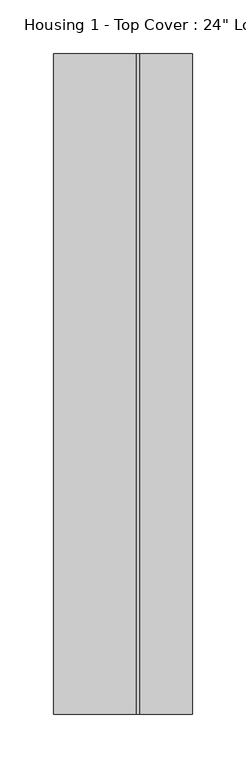
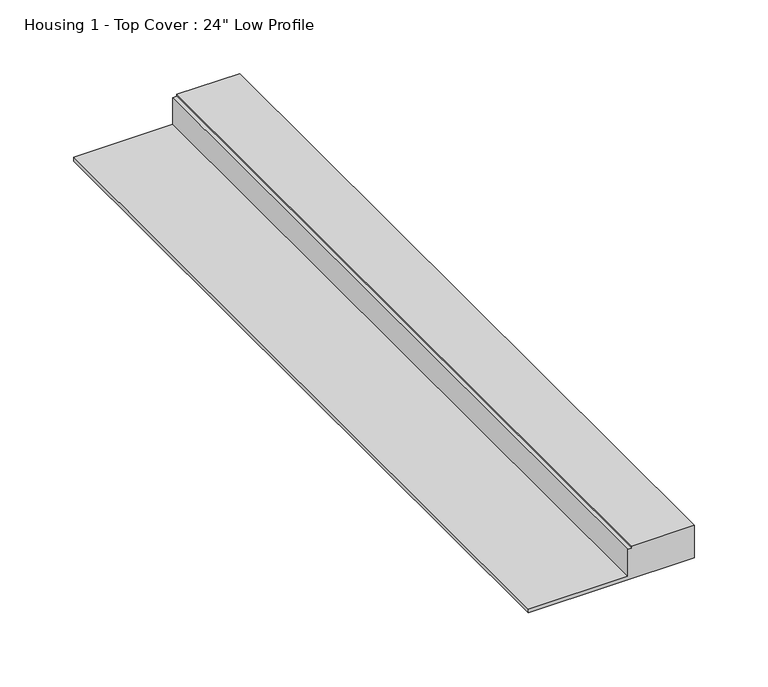
"""IFC4 building model written with IfcOpenShell, lengths in millimetres: proxy geometry."""

from ifc_helpers import new_model, si_unit, frame, origin, place, context, project, spatial, polyline, outline, extrude, source, transform, mapped, element, save


def proxy_c6f4a757(model_context):
    return source(origin(), model_context, "Body", "SweptSolid", [
        extrude(outline(polyline([(26.9875, 63.5), (26.9875, 14.2875), (25.4, 14.2875), (25.4, 11.1125), (3.175, 11.1125), (3.175, -66.675), (0.0, -66.675), (0.0, 63.5), (26.9875, 63.5)])), frame((0.0, -632.4699219, 0.0), z_axis=(0.0, 1.0, 0.0), x_axis=(0.0, 0.0, 1.0)), (0.0, 0.0, 1.0), 617.5375),
    ])


if __name__ == "__main__":
    model = new_model("IFC4")
    model_context = context("Model", 3, world=origin())
    ifc_project = project(units=[si_unit("LENGTHUNIT", "METRE", prefix="MILLI")], contexts=[model_context])
    site = spatial("IfcSite", under=ifc_project)
    building = spatial("IfcBuilding", under=site)
    placement = place(None, origin())
    proxy_shape = proxy_c6f4a757(model_context)
    element("IfcBuildingElementProxy", 1, Name="Housing 1 - Top Cover : 24\" Low Profile", ObjectType="Housing 1 - Top Cover : 24\" Low Profile", at=placement, inside=building, context=model_context, shape_type="MappedRepresentation", body=[
        mapped(proxy_shape, transform((0.0, 0.0, 0.0), x_axis=(1.0, 0.0, 0.0), y_axis=(0.0, 1.0, 0.0), z_axis=(0.0, 0.0, 1.0))),
    ])
    save(model, "model.ifc")

# Revit data of these elements
# Type "Housing 1 - Top Cover : 24\" Low Profile"
#   Type Comments = "⍁⍉⌁⌀⏭⎽⌇⍠⌜⍉⎖⌥⌦⌯⍭⏊⍻⍿⍊⏵⍊⏗⏠⍴⎡⌈⎀⍠⌓⌤⏘⎐⍀⌐⏬⏁⎈⏍⏦⎒⏬⌝⍩⍇⌣〈⎫〉⎁⏊⍥⍖⍥⍝⍦⌖⍀⏌⏭⎝⎼⏷⏞⍻⏯⎽⏷⏞⍻⏯⎽⏷⎺⌻⎝⍎⌧⏷⏟⏿⌿⍜⍦⍤⌁⍬⏶⏎⍊⏚⏉⎞⌡⎀⎪⏈⌟⌿⍾⍼⌟⌿⌢⍶⏯⏮⏭⏐⏿⍶⍷⏓⏻⎏⍶⌟⌼⏚⎹⎟⎾⏼⏢⏇⏎⎖⍭⍾⍑⍧⍭⌾⍋⍏〉⏺⍽⏙⎦⎯⎫⍲⏝⌖⏕⎲⏹⎱⎓⍪⍵⍝⌗⌗⏳⌶⎥⏗⍶⍆⏩⏙⏉⏫⌟⍻⍝⎝⎷⎳⏼⍷⍻⏻⏿"
#   URL = "http://www.metalux-lighting.com/"
#   Manufacturer = "Cooper Industries, Inc."
#   Width = 0' - 5"
#   Offset = 0' - 0"
#   Length = 2' - 0 7/16"
#   Housing Width = 0' - 2 1/16"
#   Height = 0' - 1 1/16"
#   CTRL Symbol Radius = 0' - 2 1/4"
#   CTRL Lens Offset = 0' - 0 1/16"
#   CTRL Length = 2' - 0 5/16"
#   Surface Finish [instance default] = none
#   Interior Reflective Finish [instance default] = none
#   Assembly Code = ""
# Element 1 (IfcBuildingElementProxy, "Housing 1 - Top Cover : 24\" Low Profile")
#   Surface Finish = Metal - Cooper Industries - Steel - White
#   Materials on its faces: "Metal - Cooper Industries - Steel - White"
# Materials
#   "Metal - Cooper Industries - Steel - White": class "Metal", colour RGB 244 234 229, transparency 0
